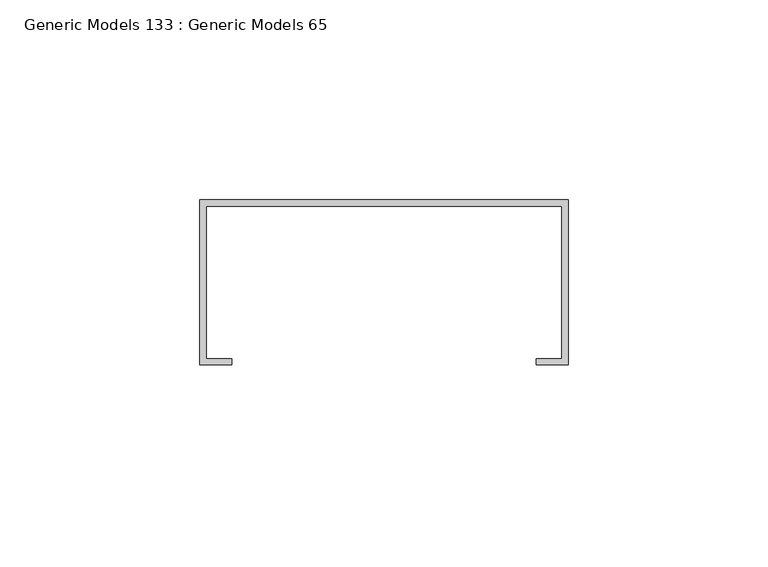
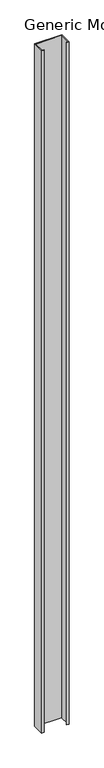
"""IFC4 building model written with IfcOpenShell, lengths in millimetres: proxy geometry, Generic Models 133 : Generic Models 65."""

from ifc_helpers import new_model, si_unit, frame, origin, place, context, project, spatial, polyline, outline, extrude, source, transform, mapped, element, save


def generic_models_133_generic_models_65_20d2f36f(model_context):
    return source(origin(), model_context, "Body", "SweptSolid", [
        extrude(outline(polyline([(45624.5985531, 630.2375), (45716.6735531, 630.2375), (45716.6735531, 588.9625), (45708.7360531, 588.9625), (45708.7360531, 590.55), (45715.0860531, 590.55), (45715.0860531, 628.65), (45626.1860531, 628.65), (45626.1860531, 590.55), (45632.5360531, 590.55), (45632.5360531, 588.9625), (45624.5985531, 588.9625), (45624.5985531, 630.2375)])), frame((0.0, 0.0, -224.388567), z_axis=(0.0, 0.0, 1.0), x_axis=(1.0, 0.0, 0.0)), (0.0, 0.0, 1.0), 2441.575),
    ])


if __name__ == "__main__":
    model = new_model("IFC4")
    model_context = context("Model", 3, world=origin())
    ifc_project = project(units=[si_unit("LENGTHUNIT", "METRE", prefix="MILLI")], contexts=[model_context])
    site = spatial("IfcSite", under=ifc_project)
    building = spatial("IfcBuilding", under=site)
    placement = place(None, origin())
    generic_models_133_generic_models_65_shape = generic_models_133_generic_models_65_20d2f36f(model_context)
    element("IfcBuildingElementProxy", 1, Name="Generic Models 133 : Generic Models 65", ObjectType="Generic Models 133 : Generic Models 65", at=placement, inside=building, context=model_context, shape_type="MappedRepresentation", body=[
        mapped(generic_models_133_generic_models_65_shape, transform((0.0, 0.0, 0.0), x_axis=(1.0, 0.0, 0.0), y_axis=(0.0, 1.0, 0.0), z_axis=(0.0, 0.0, 1.0))),
    ])
    save(model, "model.ifc")

# Revit data of these elements
# Element 1 (IfcBuildingElementProxy, "Generic Models 133 : Generic Models 65")
#   Materials on its faces: "METAL STUDS - SEE 'WALL TAG' & 'LAYER MATERIAL SCHEDULE' FOR GAUGE/SPACING & INSULATION TREATMENT, IF APPLICABLE"
# Materials
#   "METAL STUDS - SEE 'WALL TAG' & 'LAYER MATERIAL SCHEDULE' FOR GAUGE/SPACING & INSULATION TREATMENT, IF APPLICABLE": class "Unassigned", colour RGB 210 209 208, transparency 0, Keynote = "M05121300.02", Cost = 0
